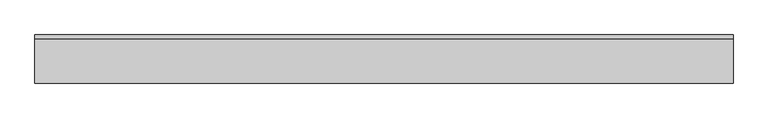
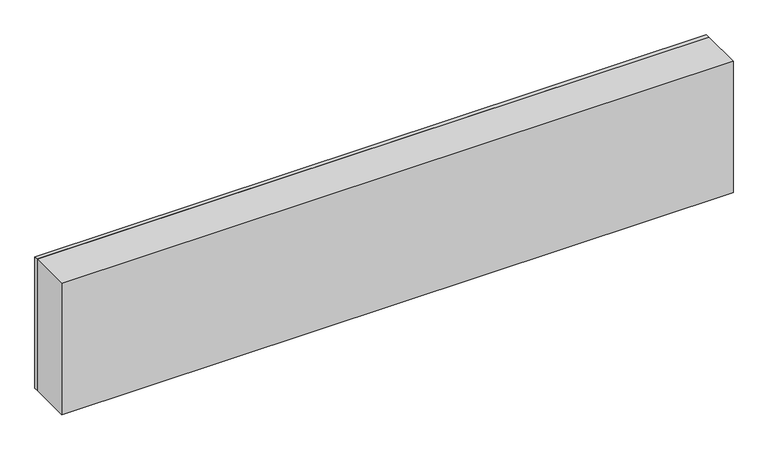
"""IFC4 building model written with IfcOpenShell, lengths in millimetres: furniture geometry, OD_CW_Upper Cabinet : OD_CW_Upper Cabinet."""

import ifcopenshell
import ifcopenshell.guid

model = None  # the IFC model being written
_history = None  # IfcOwnerHistory: only IFC2X3 demands one
_inside = {}  # id of a spatial element -> (the spatial element, [elements in it])
_under = {}  # id of a project, library or spatial element -> (it, [spatial elements below it])
_declared = {}  # id of a project -> (the project, [libraries it declares])
_typed = {}  # id of a type object -> (the type object, [elements of that type])
_made_of = {}  # id of a material, layer set ... -> (it, [elements and type objects made of it])


def new_model(schema):
    """Start an empty IFC model of exactly this schema.

    Asked for "IFC4X3", IfcOpenShell would pick the latest addendum, in which some entities
    have other attributes; the version numbers below select the first issue.
    IFC2X3 requires an IfcOwnerHistory on every rooted entity: one is made here for all.
    """
    global model, _history
    if schema == "IFC4X3":
        model = ifcopenshell.file(schema_version=(4, 3, 0, 0))
    else:
        model = ifcopenshell.file(schema=schema)
    _inside.clear()
    _under.clear()
    _declared.clear()
    _typed.clear()
    _made_of.clear()
    _history = None
    if model.schema == "IFC2X3":
        org = make("IfcOrganization", Name="unknown")
        user = make(
            "IfcPersonAndOrganization",
            ThePerson=make("IfcPerson", FamilyName="unknown"),
            TheOrganization=org,
        )
        app = make(
            "IfcApplication",
            ApplicationDeveloper=org,
            Version="unknown",
            ApplicationFullName="unknown",
            ApplicationIdentifier="unknown",
        )
        _history = make(
            "IfcOwnerHistory",
            OwningUser=user,
            OwningApplication=app,
            ChangeAction="ADDED",
            CreationDate=0,
        )
    return model


def make(cls, **values):
    """One entity of the class cls with the attributes given. An attribute that is None is left unset."""
    return model.create_entity(
        cls, **{name: value for name, value in values.items() if value is not None}
    )


def rooted(cls, **values):
    """An entity with a GlobalId (a new one), such as an element, a storey or a relation."""
    return make(cls, GlobalId=ifcopenshell.guid.new(), OwnerHistory=_history, **values)


def si_unit(unit_type, name, prefix=None):
    """IfcSIUnit, for example si_unit("LENGTHUNIT", "METRE", prefix="MILLI")."""
    return make("IfcSIUnit", UnitType=unit_type, Prefix=prefix, Name=name)


def assignment(units):
    """IfcUnitAssignment: the units of a project."""
    return None if units is None else make("IfcUnitAssignment", Units=units)


def point(xyz):
    """IfcCartesianPoint."""
    return None if xyz is None else make("IfcCartesianPoint", Coordinates=xyz)


def direction(xyz):
    """IfcDirection."""
    return None if xyz is None else make("IfcDirection", DirectionRatios=xyz)


def frame(location, z_axis=None, x_axis=None):
    """IfcAxis2Placement3D, a coordinate frame: its origin and axes. An axis left out is left unset."""
    return make(
        "IfcAxis2Placement3D",
        Location=point(location),
        Axis=direction(z_axis),
        RefDirection=direction(x_axis),
    )


def origin():
    """The frame at (0, 0, 0) with its axes left unset."""
    return frame((0.0, 0.0, 0.0))


def place(relative_to, where):
    """IfcLocalPlacement: puts the frame where relative to a parent placement (None: the world)."""
    return make(
        "IfcLocalPlacement", PlacementRelTo=relative_to, RelativePlacement=where
    )


def context(
    kind, dimensions, precision=None, world=None, true_north=None, identifier=None
):
    """IfcGeometricRepresentationContext, for example the 3D "Model" context."""
    return make(
        "IfcGeometricRepresentationContext",
        ContextIdentifier=identifier,
        ContextType=kind,
        CoordinateSpaceDimension=dimensions,
        Precision=precision,
        WorldCoordinateSystem=world,
        TrueNorth=true_north,
    )


def project(units=None, contexts=None):
    """IfcProject with its units and contexts."""
    return rooted(
        "IfcProject",
        Name="project",
        RepresentationContexts=contexts,
        UnitsInContext=assignment(units),
    )


def spatial(cls, under=None, at=None, **own):
    """A site, building, storey or space (cls), placed at a placement, below another one or the project."""
    s = rooted(cls, ObjectPlacement=at, **own)
    if under is not None:
        _under.setdefault(under.id(), (under, []))[1].append(s)
    return s


def polyline(points):
    """IfcPolyline through the points."""
    return make("IfcPolyline", Points=[point(p) for p in points])


def outline(outer, holes=None, kind="AREA"):
    """IfcArbitraryClosedProfileDef: a profile drawn as a closed curve; with holes, ...WithVoids."""
    if holes is None:
        return make("IfcArbitraryClosedProfileDef", ProfileType=kind, OuterCurve=outer)
    return make(
        "IfcArbitraryProfileDefWithVoids",
        ProfileType=kind,
        OuterCurve=outer,
        InnerCurves=holes,
    )


def extrude(swept, where, along, depth):
    """IfcExtrudedAreaSolid: the profile swept, set in the frame where, extruded along a direction by depth."""
    return make(
        "IfcExtrudedAreaSolid",
        SweptArea=swept,
        Position=where,
        ExtrudedDirection=direction(along),
        Depth=depth,
    )


def shape(context_of_items, identifier, shape_type, items):
    """IfcShapeRepresentation: the items that make up one representation, for example the "Body"."""
    return make(
        "IfcShapeRepresentation",
        ContextOfItems=context_of_items,
        RepresentationIdentifier=identifier,
        RepresentationType=shape_type,
        Items=items,
    )


def source(mapping_origin, context_of_items, identifier, shape_type, items):
    """IfcRepresentationMap: a shape defined once, which mapped items show again and again."""
    return make(
        "IfcRepresentationMap",
        MappingOrigin=mapping_origin,
        MappedRepresentation=shape(context_of_items, identifier, shape_type, items),
    )


def transform(
    local_origin,
    x_axis=None,
    y_axis=None,
    z_axis=None,
    scale=None,
    scale2=None,
    scale3=None,
    uniform=True,
):
    """IfcCartesianTransformationOperator3D, or its non-uniform kind. x_axis, y_axis, z_axis: its Axis1, 2, 3."""
    if uniform:
        return make(
            "IfcCartesianTransformationOperator3D",
            Axis1=direction(x_axis),
            Axis2=direction(y_axis),
            LocalOrigin=point(local_origin),
            Scale=scale,
            Axis3=direction(z_axis),
        )
    return make(
        "IfcCartesianTransformationOperator3DnonUniform",
        Axis1=direction(x_axis),
        Axis2=direction(y_axis),
        LocalOrigin=point(local_origin),
        Scale=scale,
        Axis3=direction(z_axis),
        Scale2=scale2,
        Scale3=scale3,
    )


def mapped(mapping_source, mapping_target):
    """IfcMappedItem: shows the shape of a source again, moved by a transform."""
    return make(
        "IfcMappedItem", MappingSource=mapping_source, MappingTarget=mapping_target
    )


def made_of(thing, what):
    """Note that an element or type object is made of a material, layer set ...; save() writes the relation."""
    if what is not None:
        _made_of.setdefault(what.id(), (what, []))[1].append(thing)
    return thing


def element(
    cls,
    number,
    at=None,
    inside=None,
    cuts=None,
    type_object=None,
    material=None,
    context=None,
    identifier="Body",
    shape_type=None,
    held_by="IfcProductDefinitionShape",
    body=None,
    shapes=None,
    **own,
):
    """One element of the class cls, such as IfcWall. Its Tag is "e" and its number.

    at: its placement. inside: the storey or other place that contains it. cuts: it is an
    opening in that element (IfcRelVoidsElement). A single representation is given by context,
    identifier, shape_type and body (its items); several are given by shapes. held_by: the class
    of the entity that holds the representations. save() writes the other relations.
    """
    e = rooted(cls, Tag="e%d" % number, ObjectPlacement=at, **own)
    if body is not None:
        shapes = [shape(context, identifier, shape_type, body)]
    if shapes is not None:
        e.Representation = make(held_by, Representations=shapes)
    if inside is not None:
        _inside.setdefault(inside.id(), (inside, []))[1].append(e)
    if cuts is not None:
        rooted(
            "IfcRelVoidsElement", RelatingBuildingElement=cuts, RelatedOpeningElement=e
        )
    if type_object is not None:
        _typed.setdefault(type_object.id(), (type_object, []))[1].append(e)
    return made_of(e, material)


def aggregate(whole, parts):
    """IfcRelAggregates: a whole, such as a stair, and the parts it consists of."""
    return rooted("IfcRelAggregates", RelatingObject=whole, RelatedObjects=parts)


def save(model, path):
    """Write the relations noted so far, then the file.

    IfcRelAggregates (storeys below a building ...), IfcRelContainedInSpatialStructure (elements
    in a storey), IfcRelDefinesByType, IfcRelAssociatesMaterial and IfcRelDeclares: one each for
    every whole, place, type object, material and project.
    """
    for whole, parts in _under.values():
        aggregate(whole, parts)
    for where, things in _inside.values():
        rooted(
            "IfcRelContainedInSpatialStructure",
            RelatedElements=things,
            RelatingStructure=where,
        )
    for kind, things in _typed.values():
        rooted("IfcRelDefinesByType", RelatedObjects=things, RelatingType=kind)
    for what, things in _made_of.values():
        rooted("IfcRelAssociatesMaterial", RelatedObjects=things, RelatingMaterial=what)
    for by, libraries in _declared.values():
        rooted("IfcRelDeclares", RelatingContext=by, RelatedDefinitions=libraries)
    model.write(path)


def furniture_746d2c86(model_context):
    return source(origin(), model_context, "Body", "SweptSolid", [
        extrude(outline(polyline([(18.7377049, -330.2), (18.7377049, -304.8), (4438.3377049, -304.8), (4438.3377049, -330.2), (18.7377049, -330.2)])), frame((0.0, 0.0, 965.2), z_axis=(0.0, 0.0, 1.0), x_axis=(1.0, 0.0, 0.0)), (0.0, 0.0, 1.0), 914.4),
        extrude(outline(polyline([(18.7377049, -609.6), (18.7377049, -330.2), (4438.3377049, -330.2), (4438.3377049, -609.6), (18.7377049, -609.6)])), frame((0.0, 0.0, 965.2), z_axis=(0.0, 0.0, 1.0), x_axis=(1.0, 0.0, 0.0)), (0.0, 0.0, 1.0), 914.4),
    ])


if __name__ == "__main__":
    model = new_model("IFC4")
    model_context = context("Model", 3, world=origin())
    ifc_project = project(units=[si_unit("LENGTHUNIT", "METRE", prefix="MILLI")], contexts=[model_context])
    site = spatial("IfcSite", under=ifc_project)
    building = spatial("IfcBuilding", under=site)
    placement = place(None, origin())
    furniture_shape = furniture_746d2c86(model_context)
    element("IfcFurniture", 1, ObjectType="OD_CW_Upper Cabinet : OD_CW_Upper Cabinet", at=placement, inside=building, context=model_context, shape_type="MappedRepresentation", body=[
        mapped(furniture_shape, transform((0.0, 0.0, 0.0), x_axis=(1.0, 0.0, 0.0), y_axis=(0.0, 1.0, 0.0), z_axis=(0.0, 0.0, 1.0))),
    ])
    save(model, "model.ifc")

# Revit data of these elements
# Type "OD_CW_Upper Cabinet : OD_CW_Upper Cabinet"
#   OD_CW_Width [instance default] = 2' - 2"
#   OD_CW_Off Floor [instance default] = 3' - 2"
#   OD_CW_Length [instance default] = 8' - 0"
#   OD_CW_Height [instance default] = 7' - 0"
#   Depth = 2' - 0"
#   Height = 3' - 0"
#   Width = 4' - 0"
#   OD_CW_Material_Front Panel [instance default] = none
# Element 1 (IfcFurniture, "OD_CW_Upper Cabinet : OD_CW_Upper Cabinet")
#   OD_CW_Width = 1' - 0"
#   OD_CW_Length = 14' - 6"
#   OD_CW_Height = 3' - 0"
#   Materials on its faces: "CASEWORK"
# Materials
#   "CASEWORK": class "Generic", colour RGB 181 181 181, transparency 0, Cost = 0
